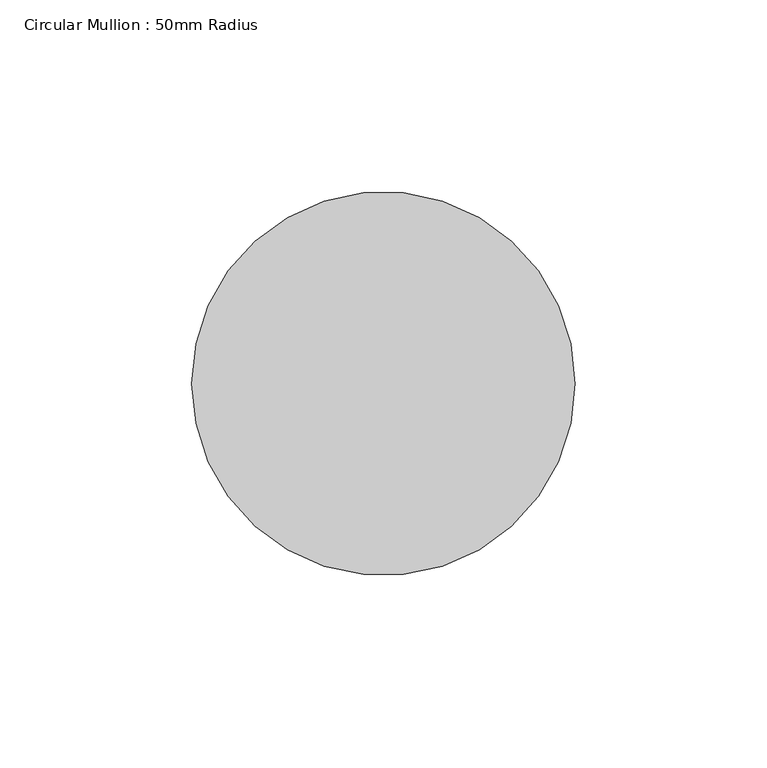
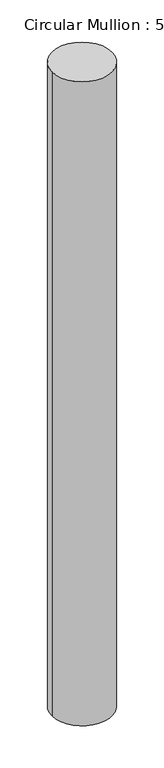
"""IFC4 building model written with IfcOpenShell, lengths in millimetres: member geometry, Circular Mullion : 50mm Radius."""

from ifc_helpers import new_model, si_unit, point, frame, origin, origin_2d, place, context, project, spatial, circle_curve, trimmed, segment, composite_curve, outline, extrude, source, transform, mapped, element, save


def circular_mullion_50mm_radius_c6c6e91c(model_context):
    return source(origin(), model_context, "Body", "SweptSolid", [
        extrude(outline(composite_curve([segment(trimmed(circle_curve(origin_2d(), 50.0), [point((50.0, 0.0))], [point((-50.0, 0.0))], False, "CARTESIAN"), True, "CONTINUOUS"), segment(trimmed(circle_curve(origin_2d(), 50.0), [point((-50.0, 0.0))], [point((50.0, 0.0))], False, "CARTESIAN"), True, "CONTINUOUS")], self_intersect=False)), frame((0.0, 0.0, -1135.6688503), z_axis=(0.0, 0.0, 1.0), x_axis=(1.0, 0.0, 0.0)), (0.0, 0.0, 1.0), 1135.6688503),
    ])


if __name__ == "__main__":
    model = new_model("IFC4")
    model_context = context("Model", 3, world=origin())
    ifc_project = project(units=[si_unit("LENGTHUNIT", "METRE", prefix="MILLI")], contexts=[model_context])
    site = spatial("IfcSite", under=ifc_project)
    building = spatial("IfcBuilding", under=site)
    placement = place(None, origin())
    circular_mullion_50mm_radius_shape = circular_mullion_50mm_radius_c6c6e91c(model_context)
    element("IfcMember", 1, ObjectType="Circular Mullion : 50mm Radius", at=placement, inside=building, context=model_context, shape_type="MappedRepresentation", body=[
        mapped(circular_mullion_50mm_radius_shape, transform((0.0, 0.0, 0.0), x_axis=(1.0, 0.0, 0.0), y_axis=(0.0, 1.0, 0.0), z_axis=(0.0, 0.0, 1.0))),
    ])
    save(model, "model.ifc")

# Revit data of these elements
# Type "Circular Mullion : 50mm Radius"
#   built-in parameter 1007350 = 0.164042 (stored number, unit not read)
# Element 1 (IfcMember, "Circular Mullion : 50mm Radius")
#   Materials on its faces: "Aluminium"
# Materials
#   "Aluminium": class "Metal", colour RGB 247 247 247, transparency 0, Description = "Aluminium 6061", Cost = 0
